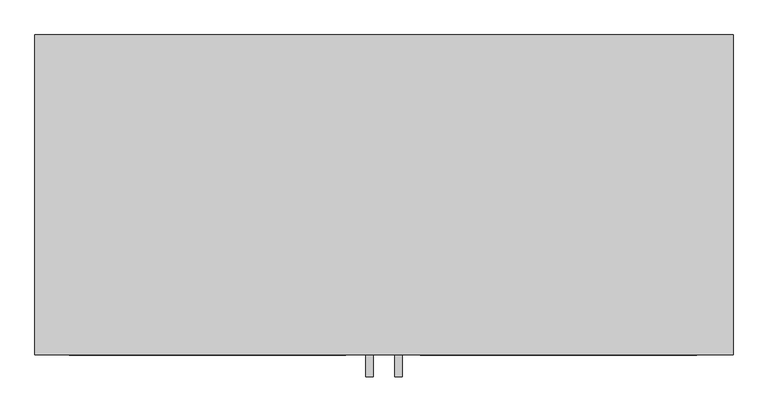
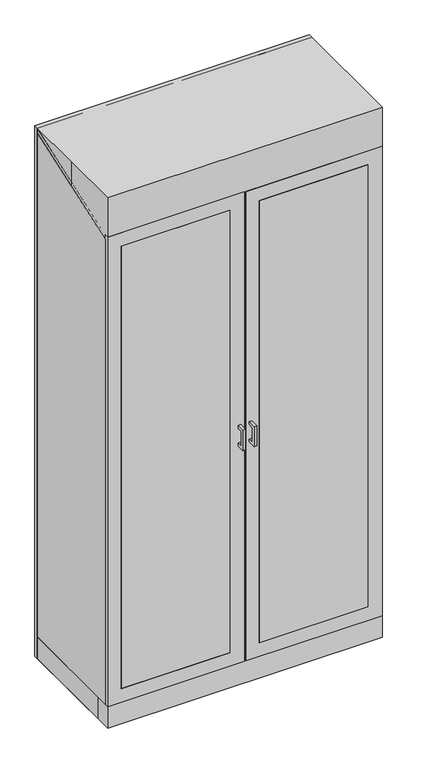
"""IFC4 building model written with IfcOpenShell, lengths in millimetres: proxy geometry, CW150 - Cabinet, Floor Standing, 5 SH, 2 GDO, ST, 98x48x22 : CW150 - Cabinet, Floor Standing, 5 SH, 2 GDO, ST, 98x48x22."""

from ifc_helpers import new_model, si_unit, frame, origin, origin_with_axes, place, context, project, spatial, polyline, outline, extrude, faceted_brep, source, transform, mapped, element, save


def specialty_equipment_dec7bf78(model_context):
    return source(origin(), model_context, "Body", "SolidModel", [
        extrude(outline(polyline([(260.35, 2467.9014525), (260.35, 101.6), (-260.35, 101.6), (-260.35, 2283.7514525), (260.35, 2467.9014525)])), frame((-609.6, 0.0, 0.0), z_axis=(1.0, 0.0, 0.0), x_axis=(0.0, 1.0, 0.0)), (0.0, 0.0, 1.0), 19.05),
        extrude(outline(polyline([(-590.55, 260.35), (-590.55, -203.2), (-609.6, -203.2), (-609.6, 260.35), (-590.55, 260.35)])), origin_with_axes(), (0.0, 0.0, 1.0), 101.6),
        extrude(outline(polyline([(609.6, 260.35), (609.6, -203.2), (590.55, -203.2), (590.55, 260.35), (609.6, 260.35)])), origin_with_axes(), (0.0, 0.0, 1.0), 101.6),
        extrude(outline(polyline([(260.35, 2467.9014525), (260.35, 101.6), (-260.35, 101.6), (-260.35, 2283.7514525), (260.35, 2467.9014525)])), frame((590.55, 0.0, 0.0), z_axis=(1.0, 0.0, 0.0), x_axis=(0.0, 1.0, 0.0)), (0.0, 0.0, 1.0), 19.05),
        extrude(outline(polyline([(546.1, -279.4), (63.5, -279.4), (63.5, -273.05), (546.1, -273.05), (546.1, -279.4)])), frame((0.0, 0.0, 165.1), z_axis=(0.0, 0.0, 1.0), x_axis=(1.0, 0.0, 0.0)), (0.0, 0.0, 1.0), 2076.45),
        extrude(outline(polyline([(-66.675, -279.4), (-549.275, -279.4), (-549.275, -273.05), (-66.675, -273.05), (-66.675, -279.4)])), frame((0.0, 0.0, 165.1), z_axis=(0.0, 0.0, 1.0), x_axis=(1.0, 0.0, 0.0)), (0.0, 0.0, 1.0), 2076.45),
        extrude(outline(polyline([(2305.05, -3.175), (2305.05, -609.6), (101.6, -609.6), (101.6, -3.175), (2305.05, -3.175)]), holes=[polyline([(2241.55, -66.675), (165.1, -66.675), (165.1, -549.275), (2241.55, -549.275), (2241.55, -66.675)])]), frame((0.0, -279.4, 0.0), z_axis=(0.0, 1.0, 0.0), x_axis=(0.0, 0.0, 1.0)), (0.0, 0.0, 1.0), 19.05),
        extrude(outline(polyline([(2305.05, 609.6), (2305.05, 3.175), (101.6, 3.175), (101.6, 609.6), (2305.05, 609.6)]), holes=[polyline([(2241.55, 546.1), (165.1, 546.1), (165.1, 63.5), (2241.55, 63.5), (2241.55, 546.1)])]), frame((0.0, -279.4, 0.0), z_axis=(0.0, 1.0, 0.0), x_axis=(0.0, 0.0, 1.0)), (0.0, 0.0, 1.0), 19.05),
        extrude(outline(polyline([(-317.4716405, 1219.2), (-279.3905468, 1219.2), (-279.3905468, 1206.5303499), (-304.8019905, 1206.5303499), (-304.8019905, 1136.6574627), (-279.3905468, 1136.6574627), (-279.3905468, 1123.9878126), (-317.4716405, 1123.9878126), (-317.4716405, 1219.2)])), frame((19.1988281, 0.0, 0.0), z_axis=(1.0, 0.0, 0.0), x_axis=(0.0, 1.0, 0.0)), (0.0, 0.0, 1.0), 12.4023438),
        extrude(outline(polyline([(590.55, -260.35), (-590.55, -260.35), (-590.55, 260.35), (590.55, 260.35), (590.55, -260.35)])), frame((0.0, 0.0, 1524.0), z_axis=(0.0, 0.0, 1.0), x_axis=(1.0, 0.0, 0.0)), (0.0, 0.0, 1.0), 25.4),
        extrude(outline(polyline([(590.55, -260.35), (-590.55, -260.35), (-590.55, 260.35), (590.55, 260.35), (590.55, -260.35)])), frame((0.0, 0.0, 1930.4), z_axis=(0.0, 0.0, 1.0), x_axis=(1.0, 0.0, 0.0)), (0.0, 0.0, 1.0), 25.4),
        extrude(outline(polyline([(590.55, -260.35), (-590.55, -260.35), (-590.55, 260.35), (590.55, 260.35), (590.55, -260.35)])), frame((0.0, 0.0, 1168.4), z_axis=(0.0, 0.0, 1.0), x_axis=(1.0, 0.0, 0.0)), (0.0, 0.0, 1.0), 25.4),
        extrude(outline(polyline([(590.55, -260.35), (-590.55, -260.35), (-590.55, 260.35), (590.55, 260.35), (590.55, -260.35)])), frame((0.0, 0.0, 800.1), z_axis=(0.0, 0.0, 1.0), x_axis=(1.0, 0.0, 0.0)), (0.0, 0.0, 1.0), 25.4),
        extrude(outline(polyline([(590.55, -260.35), (-590.55, -260.35), (-590.55, 260.35), (590.55, 260.35), (590.55, -260.35)])), frame((0.0, 0.0, 469.9), z_axis=(0.0, 0.0, 1.0), x_axis=(1.0, 0.0, 0.0)), (0.0, 0.0, 1.0), 25.4),
        faceted_brep([(-609.6, 279.4, 2489.2), (-609.6, 0.0, 2489.2), (-609.6, -279.4, 2489.2), (609.6, -279.4, 2489.2), (609.6, 279.4, 2489.2), (-609.6, 279.4, 0.0), (609.6, 279.4, 0.0), (609.6, -279.4, 0.0), (-609.6, -279.4, 0.0), (-609.6, 0.0, 0.0), (546.1, -279.4, 2241.55), (546.1, -279.4, 165.1), (63.5, -279.4, 165.1), (63.5, -279.4, 2241.55), (-66.675, -279.4, 2241.55), (-66.675, -279.4, 165.1), (-549.275, -279.4, 165.1), (-549.275, -279.4, 2241.55), (546.1, -260.35, 2241.55), (546.1, -260.35, 165.1), (63.5, -260.35, 165.1), (63.5, -260.35, 2241.55), (-66.675, -260.35, 2241.55), (-66.675, -260.35, 165.1), (-549.275, -260.35, 165.1), (-549.275, -260.35, 2241.55)], [[[0, 1, 2, 3, 4]], [[5, 6, 7, 8, 9]], [[1, 0, 5, 9]], [[2, 1, 9, 8]], [[3, 2, 8, 7], [10, 11, 12, 13], [14, 15, 16, 17]], [[4, 3, 7, 6]], [[0, 4, 6, 5]], [[10, 18, 19, 11]], [[12, 20, 21, 13]], [[11, 19, 20, 12]], [[19, 18, 21, 20]], [[18, 10, 13, 21]], [[14, 22, 23, 15]], [[16, 24, 25, 17]], [[15, 23, 24, 16]], [[23, 22, 25, 24]], [[22, 14, 17, 25]]]),
        extrude(outline(polyline([(-317.4716405, 1219.2), (-279.3905468, 1219.2), (-279.3905468, 1206.5303499), (-304.8019905, 1206.5303499), (-304.8019905, 1136.6574627), (-279.3905468, 1136.6574627), (-279.3905468, 1123.9878126), (-317.4716405, 1123.9878126), (-317.4716405, 1219.2)])), frame((-31.6011719, 0.0, 0.0), z_axis=(1.0, 0.0, 0.0), x_axis=(0.0, 1.0, 0.0)), (0.0, 0.0, 1.0), 12.4023438),
        extrude(outline(polyline([(609.6, 260.35), (-609.6, 260.35), (-609.6, 279.4), (609.6, 279.4), (609.6, 260.35)])), origin_with_axes(), (0.0, 0.0, 1.0), 2489.2),
        extrude(outline(polyline([(-260.35, 2305.05), (260.35, 2489.2), (260.35, 2467.9014525), (-260.35, 2283.7514525), (-260.35, 2305.05)])), frame((-609.6, 0.0, 0.0), z_axis=(1.0, 0.0, 0.0), x_axis=(0.0, 1.0, 0.0)), (0.0, 0.0, 1.0), 1219.2),
        extrude(outline(polyline([(590.55, -260.35), (-590.55, -260.35), (-590.55, 260.35), (590.55, 260.35), (590.55, -260.35)])), frame((0.0, 0.0, 101.6), z_axis=(0.0, 0.0, 1.0), x_axis=(1.0, 0.0, 0.0)), (0.0, 0.0, 1.0), 25.4),
        extrude(outline(polyline([(609.6, -184.15), (609.6, -203.2), (-609.6, -203.2), (-609.6, -184.15), (609.6, -184.15)])), origin_with_axes(), (0.0, 0.0, 1.0), 101.6),
    ])


if __name__ == "__main__":
    model = new_model("IFC4")
    model_context = context("Model", 3, world=origin())
    ifc_project = project(units=[si_unit("LENGTHUNIT", "METRE", prefix="MILLI")], contexts=[model_context])
    site = spatial("IfcSite", under=ifc_project)
    building = spatial("IfcBuilding", under=site)
    placement = place(None, origin())
    specialty_equipment_shape = specialty_equipment_dec7bf78(model_context)
    element("IfcBuildingElementProxy", 1, Name="CW150 - Cabinet, Floor Standing, 5 SH, 2 GDO, ST, 98x48x22 : CW150 - Cabinet, Floor Standing, 5 SH, 2 GDO, ST, 98x48x22", ObjectType="CW150 - Cabinet, Floor Standing, 5 SH, 2 GDO, ST, 98x48x22 : CW150 - Cabinet, Floor Standing, 5 SH, 2 GDO, ST, 98x48x22", at=placement, inside=building, context=model_context, shape_type="MappedRepresentation", body=[
        mapped(specialty_equipment_shape, transform((0.0, 0.0, 0.0), x_axis=(1.0, 0.0, 0.0), y_axis=(0.0, 1.0, 0.0), z_axis=(0.0, 0.0, 1.0))),
    ])
    save(model, "model.ifc")

# Revit data of these elements
# Project information
#   Room Abbreviation = "CSIA2"
#   Room Description = "Clean Workroom, Instrument Set Assembly, Medium (CSIA2)"
#   Sheets - Total = "7"
#   Project Issue Date = "Issue Date"
#   Project Status = "Project Status"
#   Client Name = "Owner"
#   Project Address = "Enter address here"
#   Project Name = "Project Name"
#   Project Number = "Project Number"
#   Publication Date = "1-Feb-16"
# Type "CW150 - Cabinet, Floor Standing, 5 SH, 2 GDO, ST, 98x48x22 : CW150 - Cabinet, Floor Standing, 5 SH, 2 GDO, ST, 98x48x22"
#   Watts2 = "0"
#   Watts1 = "0"
#   Unit_Issue = "EA"
#   UTIL_6_Misc = "-"
#   UTIL_5_NonMedGas = "-"
#   UTIL_4_MiscGas = "-"
#   UTIL_3_MedGas = "-"
#   UTIL_2_Elec = "-"
#   UTIL_1_WaterDrain = "-"
#   Nomenclature = "Cabinet, Floor Standing, 5 SH, 2 GDO, ST, 98\"x48\""
#   NSN = "6530"
#   Location [instance default] = ""
#   JSN = "CW150"
#   Fund_Source_VA = "-"
#   Fund_Source_Navy = "-"
#   Fund_Source_Army = "-"
#   Fund_Source_AF = "-"
#   ELEC_Volts2 = "0"
#   ELEC_Volts1 = "0"
#   ELEC_Phase2 = "0"
#   ELEC_Phase1 = "0"
#   ELEC_HertzSwitch = "0"
#   ELEC_HertzDependent = "0"
#   ELEC_Hertz = "0"
#   ELEC_Amps2 = "0"
#   ELEC_Amps1 = "0"
#   DetailDescription = "Floor standing storage cabinet approximately 98\" H x 48\" W x 22\" D with five adjustable shelves, framed glass hinged doors, and sloping top. Also referred to as a framed glass hinged double door case. For general purpose use throughout the facility."
#   CAT_VA = "A"
#   CAT_Navy = "A"
#   CAT_IHS = "-"
#   CAT_Army = "A"
#   CAT_AF = "A"
#   BTUperhour = "0"
#   Weight_IP = 422
#   DIM_Width_IP = 4' - 0"
#   DIM_Height_IP = 8' - 2"
#   DIM_Depth_IP = 1' - 10"
# Element 1 (IfcBuildingElementProxy, "CW150 - Cabinet, Floor Standing, 5 SH, 2 GDO, ST, 98x48x22 : CW150 - Cabinet, Floor Standing, 5 SH, 2 GDO, ST, 98x48x22")
#   Materials on its faces: "Default metal", "EquipSpace", "Glass"
# Materials
#   "Default metal": class "Unassigned", colour RGB 204 204 204, transparency 0
#   "EquipSpace": class "Unassigned", colour RGB 221 217 195, transparency 0.5
#   "Glass": class "Glass", colour RGB 0 128 192, transparency 0.75
